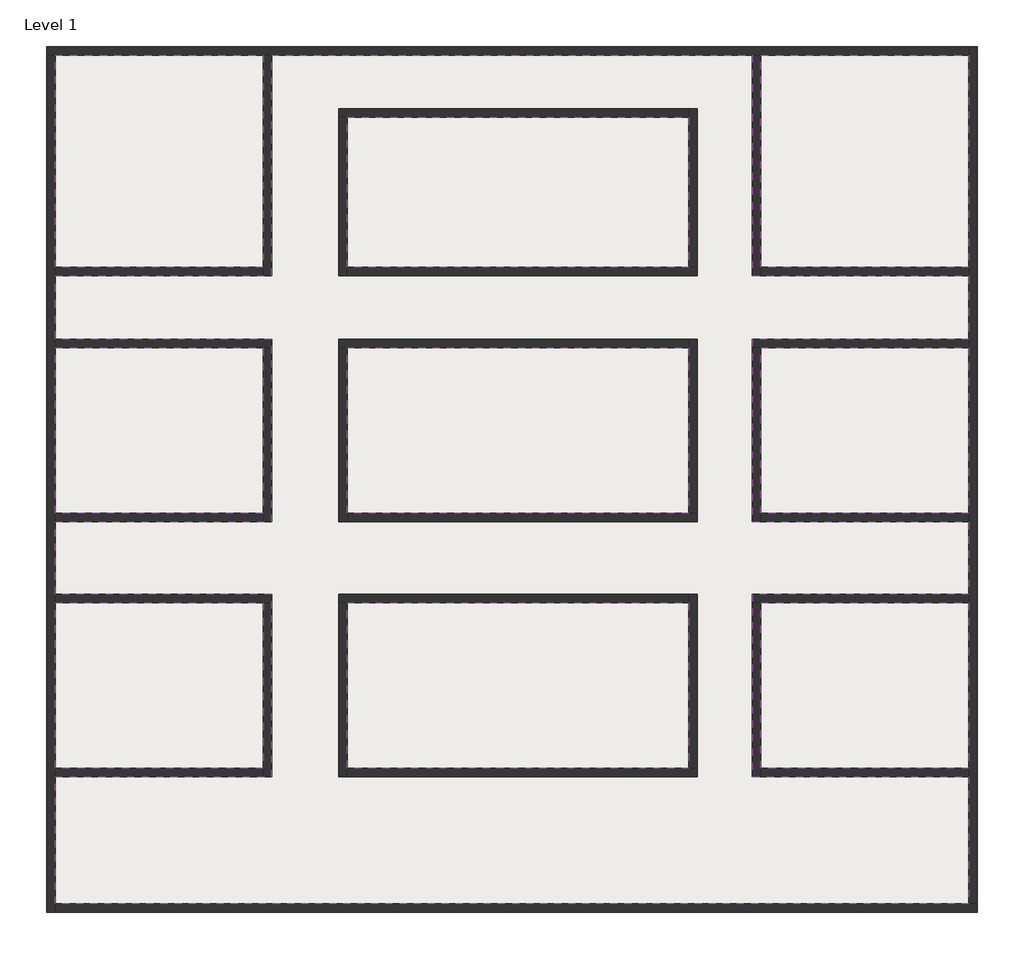
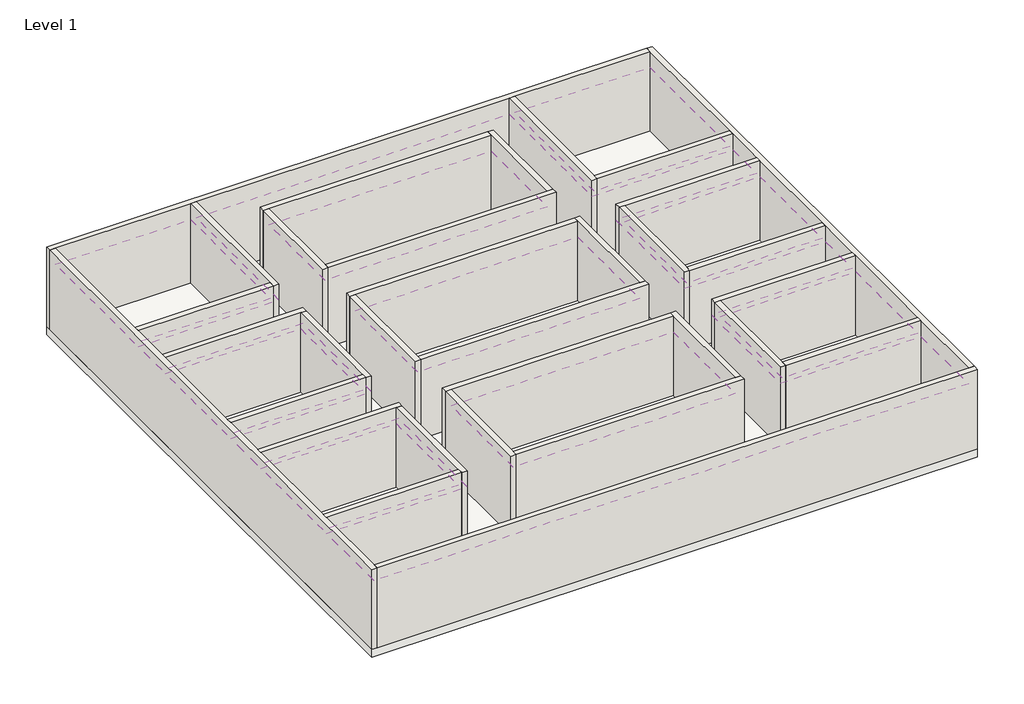
# One storey: 32 walls, 11 coverings, 1 slab.
"""IFC4 building model written with IfcOpenShell, lengths in millimetres."""

from ifc_helpers import new_model, si_unit, frame, origin, origin_with_axes, place, context, project, spatial, polyline, outline, extrude, faceted_brep, element, save

model = new_model("IFC4")

# Units and contexts
model_context = context("Model", 3, world=origin())
ifc_project = project(units=[si_unit("LENGTHUNIT", "METRE", prefix="MILLI")], contexts=[model_context])

# Site, building, storey
site = spatial("IfcSite", under=ifc_project)
building = spatial("IfcBuilding", under=site)
storey = spatial("IfcBuildingStorey", under=building, Name="Level 1", Elevation=0.0)

# Coverings
placement = place(None, origin())
element("IfcCovering", 1, ObjectType="2' x 4' ACT System", at=placement, inside=storey, context=model_context, shape_type="SweptSolid", body=[
    extrude(outline(polyline([(-11709.662063, 12460.3552234), (-6809.662063, 12460.3552234), (-6809.662063, 7460.3552234), (-11709.662063, 7460.3552234), (-11709.662063, 12460.3552234)])), frame((0.0, 0.0, 2438.4), z_axis=(0.0, 0.0, 1.0), x_axis=(1.0, 0.0, 0.0)), (0.0, 0.0, 1.0), 57.15),
])
element("IfcCovering", 2, ObjectType="2' x 4' ACT System", at=placement, inside=storey, context=model_context, shape_type="SweptSolid", body=[
    extrude(outline(polyline([(-6609.662063, 7260.3552234), (-6609.662063, 12460.3552234), (4722.664183, 12460.3552234), (4722.664183, 7260.3552234), (9822.664183, 7260.3552234), (9822.664183, 5760.3552234), (4722.664183, 5760.3552234), (4722.664183, 1460.3552234), (9822.664183, 1460.3552234), (9822.664183, -239.6447766), (4722.664183, -239.6447766), (4722.664183, -4539.6447766), (9822.664183, -4539.6447766), (9822.664183, -7539.6447766), (-11709.662063, -7539.6447766), (-11709.662063, -4539.6447766), (-6609.662063, -4539.6447766), (-6609.662063, -239.6447766), (-11709.662063, -239.6447766), (-11709.662063, 1460.3552234), (-6609.662063, 1460.3552234), (-6609.662063, 5760.3552234), (-11709.662063, 5760.3552234), (-11709.662063, 7260.3552234), (-6609.662063, 7260.3552234)]), holes=[polyline([(3422.664183, 7260.3552234), (3422.664183, 11191.3898121), (-5023.4293583, 11191.3898121), (-5023.4293583, 7260.3552234), (3422.664183, 7260.3552234)]), polyline([(3422.664183, 1460.3552234), (3422.664183, 5760.3552234), (-5023.4293583, 5760.3552234), (-5023.4293583, 1460.3552234), (3422.664183, 1460.3552234)]), polyline([(3422.664183, -4539.6447766), (3422.664183, -239.6447766), (-5023.4293583, -239.6447766), (-5023.4293583, -4539.6447766), (3422.664183, -4539.6447766)])]), frame((0.0, 0.0, 2438.4), z_axis=(0.0, 0.0, 1.0), x_axis=(1.0, 0.0, 0.0)), (0.0, 0.0, 1.0), 57.15),
])
element("IfcCovering", 3, ObjectType="2' x 4' ACT System", at=placement, inside=storey, context=model_context, shape_type="SweptSolid", body=[
    extrude(outline(polyline([(-4823.4293583, 10991.3898121), (3222.664183, 10991.3898121), (3222.664183, 7460.3552234), (-4823.4293583, 7460.3552234), (-4823.4293583, 10991.3898121)])), frame((0.0, 0.0, 2438.4), z_axis=(0.0, 0.0, 1.0), x_axis=(1.0, 0.0, 0.0)), (0.0, 0.0, 1.0), 57.15),
])
element("IfcCovering", 4, ObjectType="2' x 4' ACT System", at=placement, inside=storey, context=model_context, shape_type="SweptSolid", body=[
    extrude(outline(polyline([(4922.664183, 7460.3552234), (4922.664183, 12460.3552234), (9822.664183, 12460.3552234), (9822.664183, 7460.3552234), (4922.664183, 7460.3552234)])), frame((0.0, 0.0, 2438.4), z_axis=(0.0, 0.0, 1.0), x_axis=(1.0, 0.0, 0.0)), (0.0, 0.0, 1.0), 57.15),
])
element("IfcCovering", 5, ObjectType="2' x 4' ACT System", at=placement, inside=storey, context=model_context, shape_type="SweptSolid", body=[
    extrude(outline(polyline([(4922.664183, 5560.3552234), (9822.664183, 5560.3552234), (9822.664183, 1660.3552234), (4922.664183, 1660.3552234), (4922.664183, 5560.3552234)])), frame((0.0, 0.0, 2438.4), z_axis=(0.0, 0.0, 1.0), x_axis=(1.0, 0.0, 0.0)), (0.0, 0.0, 1.0), 57.15),
])
element("IfcCovering", 6, ObjectType="2' x 4' ACT System", at=placement, inside=storey, context=model_context, shape_type="SweptSolid", body=[
    extrude(outline(polyline([(4922.664183, -439.6447766), (9822.664183, -439.6447766), (9822.664183, -4339.6447766), (4922.664183, -4339.6447766), (4922.664183, -439.6447766)])), frame((0.0, 0.0, 2438.4), z_axis=(0.0, 0.0, 1.0), x_axis=(1.0, 0.0, 0.0)), (0.0, 0.0, 1.0), 57.15),
])
element("IfcCovering", 7, ObjectType="2' x 4' ACT System", at=placement, inside=storey, context=model_context, shape_type="SweptSolid", body=[
    extrude(outline(polyline([(-4823.4293583, -439.6447766), (3222.664183, -439.6447766), (3222.664183, -4339.6447766), (-4823.4293583, -4339.6447766), (-4823.4293583, -439.6447766)])), frame((0.0, 0.0, 2438.4), z_axis=(0.0, 0.0, 1.0), x_axis=(1.0, 0.0, 0.0)), (0.0, 0.0, 1.0), 57.15),
])
element("IfcCovering", 8, ObjectType="2' x 4' ACT System", at=placement, inside=storey, context=model_context, shape_type="SweptSolid", body=[
    extrude(outline(polyline([(-11709.662063, -4339.6447766), (-11709.662063, -439.6447766), (-6809.662063, -439.6447766), (-6809.662063, -4339.6447766), (-11709.662063, -4339.6447766)])), frame((0.0, 0.0, 2438.4), z_axis=(0.0, 0.0, 1.0), x_axis=(1.0, 0.0, 0.0)), (0.0, 0.0, 1.0), 57.15),
])
element("IfcCovering", 9, ObjectType="2' x 4' ACT System", at=placement, inside=storey, context=model_context, shape_type="SweptSolid", body=[
    extrude(outline(polyline([(-11709.662063, 1660.3552234), (-11709.662063, 5560.3552234), (-6809.662063, 5560.3552234), (-6809.662063, 1660.3552234), (-11709.662063, 1660.3552234)])), frame((0.0, 0.0, 2438.4), z_axis=(0.0, 0.0, 1.0), x_axis=(1.0, 0.0, 0.0)), (0.0, 0.0, 1.0), 57.15),
])
element("IfcCovering", 10, ObjectType="2' x 4' ACT System", at=placement, inside=storey, context=model_context, shape_type="SweptSolid", body=[
    extrude(outline(polyline([(-4823.4293583, 5560.3552234), (3222.664183, 5560.3552234), (3222.664183, 1660.3552234), (-4823.4293583, 1660.3552234), (-4823.4293583, 5560.3552234)])), frame((0.0, 0.0, 2438.4), z_axis=(0.0, 0.0, 1.0), x_axis=(1.0, 0.0, 0.0)), (0.0, 0.0, 1.0), 57.15),
])
element("IfcCovering", 11, ObjectType="2' x 4' ACT System", at=placement, inside=storey, context=model_context, shape_type="SweptSolid", body=[
    extrude(outline(polyline([(4922.664183, 5560.3552234), (9822.664183, 5560.3552234), (9822.664183, 1660.3552234), (4922.664183, 1660.3552234), (4922.664183, 5560.3552234)])), frame((0.0, 0.0, 2438.4), z_axis=(0.0, 0.0, 1.0), x_axis=(1.0, 0.0, 0.0)), (0.0, 0.0, 1.0), 57.15),
])

# Slab
element("IfcSlab", 12, ObjectType="Generic - 12\"", at=placement, inside=storey, context=model_context, shape_type="SweptSolid", body=[
    extrude(outline(polyline([(10022.664183, 12660.3552234), (10022.664183, -7739.6447766), (-11909.662063, -7739.6447766), (-11909.662063, 12660.3552234), (10022.664183, 12660.3552234)])), frame((0.0, 0.0, -304.8), z_axis=(0.0, 0.0, 1.0), x_axis=(1.0, 0.0, 0.0)), (0.0, 0.0, 1.0), 304.8),
])

# Walls
element("IfcWall", 13, ObjectType="Generic - 200mm", at=placement, inside=storey, context=model_context, shape_type="Brep", body=[
    faceted_brep([(-11909.662063, 12460.3552234, 0.0), (-11709.662063, 12460.3552234, 0.0), (-6809.662063, 12460.3552234, 0.0), (-6609.662063, 12460.3552234, 0.0), (4722.664183, 12460.3552234, 0.0), (4922.664183, 12460.3552234, 0.0), (9822.664183, 12460.3552234, 0.0), (9822.664183, 12460.3552234, 3048.0), (4922.664183, 12460.3552234, 3048.0), (4722.664183, 12460.3552234, 3048.0), (-6609.662063, 12460.3552234, 3048.0), (-6809.662063, 12460.3552234, 3048.0), (-11709.662063, 12460.3552234, 3048.0), (-11909.662063, 12460.3552234, 3048.0), (-11909.662063, 12660.3552234, 0.0), (-11909.662063, 12660.3552234, 3048.0), (9822.664183, 12660.3552234, 3048.0), (9822.664183, 12660.3552234, 0.0)], [[[0, 1, 2, 3, 4, 5, 6, 7, 8, 9, 10, 11, 12, 13]], [[14, 15, 16, 17]], [[6, 5, 4, 3, 2, 1, 0, 14, 17]], [[0, 13, 15, 14]], [[7, 6, 17, 16]], [[13, 12, 11, 10, 9, 8, 7, 16, 15]]]),
])
element("IfcWall", 14, ObjectType="Generic - 200mm", at=placement, inside=storey, context=model_context, shape_type="Brep", body=[
    faceted_brep([(-11709.662063, -7739.6447766, 0.0), (-11709.662063, -7539.6447766, 0.0), (-11709.662063, -4539.6447766, 0.0), (-11709.662063, -4339.6447766, 0.0), (-11709.662063, -439.6447766, 0.0), (-11709.662063, -239.6447766, 0.0), (-11709.662063, 1460.3552234, 0.0), (-11709.662063, 1660.3552234, 0.0), (-11709.662063, 5560.3552234, 0.0), (-11709.662063, 5760.3552234, 0.0), (-11709.662063, 7260.3552234, 0.0), (-11709.662063, 7460.3552234, 0.0), (-11709.662063, 12460.3552234, 0.0), (-11709.662063, 12460.3552234, 3048.0), (-11709.662063, 7460.3552234, 3048.0), (-11709.662063, 7260.3552234, 3048.0), (-11709.662063, 5760.3552234, 3048.0), (-11709.662063, 5560.3552234, 3048.0), (-11709.662063, 1660.3552234, 3048.0), (-11709.662063, 1460.3552234, 3048.0), (-11709.662063, -239.6447766, 3048.0), (-11709.662063, -439.6447766, 3048.0), (-11709.662063, -4339.6447766, 3048.0), (-11709.662063, -4539.6447766, 3048.0), (-11709.662063, -7539.6447766, 3048.0), (-11709.662063, -7739.6447766, 3048.0), (-11909.662063, -7739.6447766, 0.0), (-11909.662063, -7739.6447766, 3048.0), (-11909.662063, 12460.3552234, 3048.0), (-11909.662063, 12460.3552234, 0.0)], [[[0, 1, 2, 3, 4, 5, 6, 7, 8, 9, 10, 11, 12, 13, 14, 15, 16, 17, 18, 19, 20, 21, 22, 23, 24, 25]], [[26, 27, 28, 29]], [[12, 11, 10, 9, 8, 7, 6, 5, 4, 3, 2, 1, 0, 26, 29]], [[0, 25, 27, 26]], [[13, 12, 29, 28]], [[25, 24, 23, 22, 21, 20, 19, 18, 17, 16, 15, 14, 13, 28, 27]]]),
])
element("IfcWall", 15, ObjectType="Generic - 200mm", at=placement, inside=storey, context=model_context, shape_type="Brep", body=[
    faceted_brep([(10022.664183, -7539.6447766, 0.0), (9822.664183, -7539.6447766, 0.0), (-11709.662063, -7539.6447766, 0.0), (-11709.662063, -7539.6447766, 3048.0), (9822.664183, -7539.6447766, 3048.0), (10022.664183, -7539.6447766, 3048.0), (10022.664183, -7739.6447766, 0.0), (10022.664183, -7739.6447766, 3048.0), (-11709.662063, -7739.6447766, 3048.0), (-11709.662063, -7739.6447766, 0.0)], [[[0, 1, 2, 3, 4, 5]], [[6, 7, 8, 9]], [[2, 1, 0, 6, 9]], [[0, 5, 7, 6]], [[3, 2, 9, 8]], [[5, 4, 3, 8, 7]]]),
])
element("IfcWall", 16, ObjectType="Generic - 200mm", at=placement, inside=storey, context=model_context, shape_type="Brep", body=[
    faceted_brep([(9822.664183, 12660.3552234, 0.0), (9822.664183, 12460.3552234, 0.0), (9822.664183, 7460.3552234, 0.0), (9822.664183, 7260.3552234, 0.0), (9822.664183, 5760.3552234, 0.0), (9822.664183, 5560.3552234, 0.0), (9822.664183, 1660.3552234, 0.0), (9822.664183, 1460.3552234, 0.0), (9822.664183, -239.6447766, 0.0), (9822.664183, -439.6447766, 0.0), (9822.664183, -4339.6447766, 0.0), (9822.664183, -4539.6447766, 0.0), (9822.664183, -7539.6447766, 0.0), (9822.664183, -7539.6447766, 3048.0), (9822.664183, -4539.6447766, 3048.0), (9822.664183, -4339.6447766, 3048.0), (9822.664183, -439.6447766, 3048.0), (9822.664183, -239.6447766, 3048.0), (9822.664183, 1460.3552234, 3048.0), (9822.664183, 1660.3552234, 3048.0), (9822.664183, 5560.3552234, 3048.0), (9822.664183, 5760.3552234, 3048.0), (9822.664183, 7260.3552234, 3048.0), (9822.664183, 7460.3552234, 3048.0), (9822.664183, 12460.3552234, 3048.0), (9822.664183, 12660.3552234, 3048.0), (10022.664183, 12660.3552234, 0.0), (10022.664183, 12660.3552234, 3048.0), (10022.664183, -7539.6447766, 3048.0), (10022.664183, -7539.6447766, 0.0)], [[[0, 1, 2, 3, 4, 5, 6, 7, 8, 9, 10, 11, 12, 13, 14, 15, 16, 17, 18, 19, 20, 21, 22, 23, 24, 25]], [[26, 27, 28, 29]], [[12, 11, 10, 9, 8, 7, 6, 5, 4, 3, 2, 1, 0, 26, 29]], [[0, 25, 27, 26]], [[13, 12, 29, 28]], [[25, 24, 23, 22, 21, 20, 19, 18, 17, 16, 15, 14, 13, 28, 27]]]),
])
element("IfcWall", 17, ObjectType="Generic - 200mm", at=placement, inside=storey, context=model_context, shape_type="Brep", body=[
    faceted_brep([(-6809.662063, -439.6447766, 0.0), (-6809.662063, -4339.6447766, 0.0), (-6809.662063, -4539.6447766, 0.0), (-6809.662063, -4539.6447766, 3048.0), (-6809.662063, -4339.6447766, 3048.0), (-6809.662063, -439.6447766, 3048.0), (-6609.662063, -439.6447766, 0.0), (-6609.662063, -439.6447766, 3048.0), (-6609.662063, -4539.6447766, 3048.0), (-6609.662063, -4539.6447766, 0.0)], [[[0, 1, 2, 3, 4, 5]], [[6, 7, 8, 9]], [[2, 1, 0, 6, 9]], [[3, 2, 9, 8]], [[0, 5, 7, 6]], [[5, 4, 3, 8, 7]]]),
])
element("IfcWall", 18, ObjectType="Generic - 200mm", at=placement, inside=storey, context=model_context, shape_type="SweptSolid", body=[
    extrude(outline(polyline([(-11709.662063, -4339.6447766), (-6809.662063, -4339.6447766), (-6809.662063, -4539.6447766), (-11709.662063, -4539.6447766), (-11709.662063, -4339.6447766)])), origin_with_axes(), (0.0, 0.0, 1.0), 3048.0),
])
element("IfcWall", 19, ObjectType="Generic - 200mm", at=placement, inside=storey, context=model_context, shape_type="Brep", body=[
    faceted_brep([(-11709.662063, -439.6447766, 0.0), (-6809.662063, -439.6447766, 0.0), (-6609.662063, -439.6447766, 0.0), (-6609.662063, -439.6447766, 3048.0), (-6809.662063, -439.6447766, 3048.0), (-11709.662063, -439.6447766, 3048.0), (-11709.662063, -239.6447766, 0.0), (-11709.662063, -239.6447766, 3048.0), (-6609.662063, -239.6447766, 3048.0), (-6609.662063, -239.6447766, 0.0)], [[[0, 1, 2, 3, 4, 5]], [[6, 7, 8, 9]], [[2, 1, 0, 6, 9]], [[0, 5, 7, 6]], [[3, 2, 9, 8]], [[5, 4, 3, 8, 7]]]),
])
element("IfcWall", 20, ObjectType="Generic - 200mm", at=placement, inside=storey, context=model_context, shape_type="Brep", body=[
    faceted_brep([(-6809.662063, 5560.3552234, 0.0), (-6809.662063, 1660.3552234, 0.0), (-6809.662063, 1460.3552234, 0.0), (-6809.662063, 1460.3552234, 3048.0), (-6809.662063, 1660.3552234, 3048.0), (-6809.662063, 5560.3552234, 3048.0), (-6609.662063, 5560.3552234, 0.0), (-6609.662063, 5560.3552234, 3048.0), (-6609.662063, 1460.3552234, 3048.0), (-6609.662063, 1460.3552234, 0.0)], [[[0, 1, 2, 3, 4, 5]], [[6, 7, 8, 9]], [[2, 1, 0, 6, 9]], [[3, 2, 9, 8]], [[0, 5, 7, 6]], [[5, 4, 3, 8, 7]]]),
])
element("IfcWall", 21, ObjectType="Generic - 200mm", at=placement, inside=storey, context=model_context, shape_type="SweptSolid", body=[
    extrude(outline(polyline([(-11709.662063, 1660.3552234), (-6809.662063, 1660.3552234), (-6809.662063, 1460.3552234), (-11709.662063, 1460.3552234), (-11709.662063, 1660.3552234)])), origin_with_axes(), (0.0, 0.0, 1.0), 3048.0),
])
element("IfcWall", 22, ObjectType="Generic - 200mm", at=placement, inside=storey, context=model_context, shape_type="Brep", body=[
    faceted_brep([(-11709.662063, 5560.3552234, 0.0), (-6809.662063, 5560.3552234, 0.0), (-6609.662063, 5560.3552234, 0.0), (-6609.662063, 5560.3552234, 3048.0), (-6809.662063, 5560.3552234, 3048.0), (-11709.662063, 5560.3552234, 3048.0), (-11709.662063, 5760.3552234, 0.0), (-11709.662063, 5760.3552234, 3048.0), (-6609.662063, 5760.3552234, 3048.0), (-6609.662063, 5760.3552234, 0.0)], [[[0, 1, 2, 3, 4, 5]], [[6, 7, 8, 9]], [[2, 1, 0, 6, 9]], [[3, 2, 9, 8]], [[0, 5, 7, 6]], [[5, 4, 3, 8, 7]]]),
])
element("IfcWall", 23, ObjectType="Generic - 200mm", at=placement, inside=storey, context=model_context, shape_type="Brep", body=[
    faceted_brep([(-6809.662063, 12460.3552234, 0.0), (-6809.662063, 7460.3552234, 0.0), (-6809.662063, 7260.3552234, 0.0), (-6809.662063, 7260.3552234, 3048.0), (-6809.662063, 7460.3552234, 3048.0), (-6809.662063, 12460.3552234, 3048.0), (-6609.662063, 12460.3552234, 0.0), (-6609.662063, 12460.3552234, 3048.0), (-6609.662063, 7260.3552234, 3048.0), (-6609.662063, 7260.3552234, 0.0)], [[[0, 1, 2, 3, 4, 5]], [[6, 7, 8, 9]], [[2, 1, 0, 6, 9]], [[3, 2, 9, 8]], [[0, 5, 7, 6]], [[5, 4, 3, 8, 7]]]),
])
element("IfcWall", 24, ObjectType="Generic - 200mm", at=placement, inside=storey, context=model_context, shape_type="SweptSolid", body=[
    extrude(outline(polyline([(-11709.662063, 7460.3552234), (-6809.662063, 7460.3552234), (-6809.662063, 7260.3552234), (-11709.662063, 7260.3552234), (-11709.662063, 7460.3552234)])), origin_with_axes(), (0.0, 0.0, 1.0), 3048.0),
])
element("IfcWall", 25, ObjectType="Generic - 200mm", at=placement, inside=storey, context=model_context, shape_type="Brep", body=[
    faceted_brep([(-5023.4293583, 10991.3898121, 0.0), (-4823.4293583, 10991.3898121, 0.0), (3222.664183, 10991.3898121, 0.0), (3222.664183, 10991.3898121, 3048.0), (-4823.4293583, 10991.3898121, 3048.0), (-5023.4293583, 10991.3898121, 3048.0), (-5023.4293583, 11191.3898121, 0.0), (-5023.4293583, 11191.3898121, 3048.0), (3222.664183, 11191.3898121, 3048.0), (3222.664183, 11191.3898121, 0.0)], [[[0, 1, 2, 3, 4, 5]], [[6, 7, 8, 9]], [[2, 1, 0, 6, 9]], [[0, 5, 7, 6]], [[3, 2, 9, 8]], [[5, 4, 3, 8, 7]]]),
])
element("IfcWall", 26, ObjectType="Generic - 200mm", at=placement, inside=storey, context=model_context, shape_type="Brep", body=[
    faceted_brep([(-4823.4293583, 7260.3552234, 0.0), (-4823.4293583, 7460.3552234, 0.0), (-4823.4293583, 10991.3898121, 0.0), (-4823.4293583, 10991.3898121, 3048.0), (-4823.4293583, 7460.3552234, 3048.0), (-4823.4293583, 7260.3552234, 3048.0), (-5023.4293583, 7260.3552234, 0.0), (-5023.4293583, 7260.3552234, 3048.0), (-5023.4293583, 10991.3898121, 3048.0), (-5023.4293583, 10991.3898121, 0.0)], [[[0, 1, 2, 3, 4, 5]], [[6, 7, 8, 9]], [[2, 1, 0, 6, 9]], [[0, 5, 7, 6]], [[3, 2, 9, 8]], [[5, 4, 3, 8, 7]]]),
])
element("IfcWall", 27, ObjectType="Generic - 200mm", at=placement, inside=storey, context=model_context, shape_type="Brep", body=[
    faceted_brep([(3422.664183, 7460.3552234, 0.0), (3222.664183, 7460.3552234, 0.0), (-4823.4293583, 7460.3552234, 0.0), (-4823.4293583, 7460.3552234, 3048.0), (3222.664183, 7460.3552234, 3048.0), (3422.664183, 7460.3552234, 3048.0), (3422.664183, 7260.3552234, 0.0), (3422.664183, 7260.3552234, 3048.0), (-4823.4293583, 7260.3552234, 3048.0), (-4823.4293583, 7260.3552234, 0.0)], [[[0, 1, 2, 3, 4, 5]], [[6, 7, 8, 9]], [[2, 1, 0, 6, 9]], [[0, 5, 7, 6]], [[3, 2, 9, 8]], [[5, 4, 3, 8, 7]]]),
])
element("IfcWall", 28, ObjectType="Generic - 200mm", at=placement, inside=storey, context=model_context, shape_type="Brep", body=[
    faceted_brep([(3222.664183, 11191.3898121, 0.0), (3222.664183, 10991.3898121, 0.0), (3222.664183, 7460.3552234, 0.0), (3222.664183, 7460.3552234, 3048.0), (3222.664183, 10991.3898121, 3048.0), (3222.664183, 11191.3898121, 3048.0), (3422.664183, 11191.3898121, 0.0), (3422.664183, 11191.3898121, 3048.0), (3422.664183, 7460.3552234, 3048.0), (3422.664183, 7460.3552234, 0.0)], [[[0, 1, 2, 3, 4, 5]], [[6, 7, 8, 9]], [[2, 1, 0, 6, 9]], [[0, 5, 7, 6]], [[3, 2, 9, 8]], [[5, 4, 3, 8, 7]]]),
])
element("IfcWall", 29, ObjectType="Generic - 200mm", at=placement, inside=storey, context=model_context, shape_type="Brep", body=[
    faceted_brep([(-5023.4293583, 5560.3552234, 0.0), (-4823.4293583, 5560.3552234, 0.0), (3222.664183, 5560.3552234, 0.0), (3222.664183, 5560.3552234, 3048.0), (-4823.4293583, 5560.3552234, 3048.0), (-5023.4293583, 5560.3552234, 3048.0), (-5023.4293583, 5760.3552234, 0.0), (-5023.4293583, 5760.3552234, 3048.0), (3222.664183, 5760.3552234, 3048.0), (3222.664183, 5760.3552234, 0.0)], [[[0, 1, 2, 3, 4, 5]], [[6, 7, 8, 9]], [[2, 1, 0, 6, 9]], [[0, 5, 7, 6]], [[3, 2, 9, 8]], [[5, 4, 3, 8, 7]]]),
])
element("IfcWall", 30, ObjectType="Generic - 200mm", at=placement, inside=storey, context=model_context, shape_type="Brep", body=[
    faceted_brep([(-4823.4293583, 1460.3552234, 0.0), (-4823.4293583, 1660.3552234, 0.0), (-4823.4293583, 5560.3552234, 0.0), (-4823.4293583, 5560.3552234, 3048.0), (-4823.4293583, 1660.3552234, 3048.0), (-4823.4293583, 1460.3552234, 3048.0), (-5023.4293583, 1460.3552234, 0.0), (-5023.4293583, 1460.3552234, 3048.0), (-5023.4293583, 5560.3552234, 3048.0), (-5023.4293583, 5560.3552234, 0.0)], [[[0, 1, 2, 3, 4, 5]], [[6, 7, 8, 9]], [[2, 1, 0, 6, 9]], [[0, 5, 7, 6]], [[3, 2, 9, 8]], [[5, 4, 3, 8, 7]]]),
])
element("IfcWall", 31, ObjectType="Generic - 200mm", at=placement, inside=storey, context=model_context, shape_type="Brep", body=[
    faceted_brep([(3422.664183, 1660.3552234, 0.0), (3222.664183, 1660.3552234, 0.0), (-4823.4293583, 1660.3552234, 0.0), (-4823.4293583, 1660.3552234, 3048.0), (3222.664183, 1660.3552234, 3048.0), (3422.664183, 1660.3552234, 3048.0), (3422.664183, 1460.3552234, 0.0), (3422.664183, 1460.3552234, 3048.0), (-4823.4293583, 1460.3552234, 3048.0), (-4823.4293583, 1460.3552234, 0.0)], [[[0, 1, 2, 3, 4, 5]], [[6, 7, 8, 9]], [[2, 1, 0, 6, 9]], [[0, 5, 7, 6]], [[3, 2, 9, 8]], [[5, 4, 3, 8, 7]]]),
])
element("IfcWall", 32, ObjectType="Generic - 200mm", at=placement, inside=storey, context=model_context, shape_type="Brep", body=[
    faceted_brep([(3222.664183, 5760.3552234, 0.0), (3222.664183, 5560.3552234, 0.0), (3222.664183, 1660.3552234, 0.0), (3222.664183, 1660.3552234, 3048.0), (3222.664183, 5560.3552234, 3048.0), (3222.664183, 5760.3552234, 3048.0), (3422.664183, 5760.3552234, 0.0), (3422.664183, 5760.3552234, 3048.0), (3422.664183, 1660.3552234, 3048.0), (3422.664183, 1660.3552234, 0.0)], [[[0, 1, 2, 3, 4, 5]], [[6, 7, 8, 9]], [[2, 1, 0, 6, 9]], [[0, 5, 7, 6]], [[3, 2, 9, 8]], [[5, 4, 3, 8, 7]]]),
])
element("IfcWall", 33, ObjectType="Generic - 200mm", at=placement, inside=storey, context=model_context, shape_type="Brep", body=[
    faceted_brep([(-5023.4293583, -439.6447766, 0.0), (-4823.4293583, -439.6447766, 0.0), (3222.664183, -439.6447766, 0.0), (3222.664183, -439.6447766, 3048.0), (-4823.4293583, -439.6447766, 3048.0), (-5023.4293583, -439.6447766, 3048.0), (-5023.4293583, -239.6447766, 0.0), (-5023.4293583, -239.6447766, 3048.0), (3222.664183, -239.6447766, 3048.0), (3222.664183, -239.6447766, 0.0)], [[[0, 1, 2, 3, 4, 5]], [[6, 7, 8, 9]], [[2, 1, 0, 6, 9]], [[0, 5, 7, 6]], [[3, 2, 9, 8]], [[5, 4, 3, 8, 7]]]),
])
element("IfcWall", 34, ObjectType="Generic - 200mm", at=placement, inside=storey, context=model_context, shape_type="Brep", body=[
    faceted_brep([(-4823.4293583, -4539.6447766, 0.0), (-4823.4293583, -4339.6447766, 0.0), (-4823.4293583, -439.6447766, 0.0), (-4823.4293583, -439.6447766, 3048.0), (-4823.4293583, -4339.6447766, 3048.0), (-4823.4293583, -4539.6447766, 3048.0), (-5023.4293583, -4539.6447766, 0.0), (-5023.4293583, -4539.6447766, 3048.0), (-5023.4293583, -439.6447766, 3048.0), (-5023.4293583, -439.6447766, 0.0)], [[[0, 1, 2, 3, 4, 5]], [[6, 7, 8, 9]], [[2, 1, 0, 6, 9]], [[0, 5, 7, 6]], [[3, 2, 9, 8]], [[5, 4, 3, 8, 7]]]),
])
element("IfcWall", 35, ObjectType="Generic - 200mm", at=placement, inside=storey, context=model_context, shape_type="Brep", body=[
    faceted_brep([(3422.664183, -4339.6447766, 0.0), (3222.664183, -4339.6447766, 0.0), (-4823.4293583, -4339.6447766, 0.0), (-4823.4293583, -4339.6447766, 3048.0), (3222.664183, -4339.6447766, 3048.0), (3422.664183, -4339.6447766, 3048.0), (3422.664183, -4539.6447766, 0.0), (3422.664183, -4539.6447766, 3048.0), (-4823.4293583, -4539.6447766, 3048.0), (-4823.4293583, -4539.6447766, 0.0)], [[[0, 1, 2, 3, 4, 5]], [[6, 7, 8, 9]], [[2, 1, 0, 6, 9]], [[0, 5, 7, 6]], [[3, 2, 9, 8]], [[5, 4, 3, 8, 7]]]),
])
element("IfcWall", 36, ObjectType="Generic - 200mm", at=placement, inside=storey, context=model_context, shape_type="Brep", body=[
    faceted_brep([(3222.664183, -239.6447766, 0.0), (3222.664183, -439.6447766, 0.0), (3222.664183, -4339.6447766, 0.0), (3222.664183, -4339.6447766, 3048.0), (3222.664183, -439.6447766, 3048.0), (3222.664183, -239.6447766, 3048.0), (3422.664183, -239.6447766, 0.0), (3422.664183, -239.6447766, 3048.0), (3422.664183, -4339.6447766, 3048.0), (3422.664183, -4339.6447766, 0.0)], [[[0, 1, 2, 3, 4, 5]], [[6, 7, 8, 9]], [[2, 1, 0, 6, 9]], [[0, 5, 7, 6]], [[3, 2, 9, 8]], [[5, 4, 3, 8, 7]]]),
])
element("IfcWall", 37, ObjectType="Generic - 200mm", at=placement, inside=storey, context=model_context, shape_type="Brep", body=[
    faceted_brep([(4722.664183, -439.6447766, 0.0), (4722.664183, -4539.6447766, 0.0), (4722.664183, -4539.6447766, 3048.0), (4722.664183, -439.6447766, 3048.0), (4922.664183, -439.6447766, 0.0), (4922.664183, -439.6447766, 3048.0), (4922.664183, -4339.6447766, 3048.0), (4922.664183, -4539.6447766, 3048.0), (4922.664183, -4539.6447766, 0.0), (4922.664183, -4339.6447766, 0.0)], [[[0, 1, 2, 3]], [[4, 5, 6, 7, 8, 9]], [[1, 0, 4, 9, 8]], [[2, 1, 8, 7]], [[0, 3, 5, 4]], [[3, 2, 7, 6, 5]]]),
])
element("IfcWall", 38, ObjectType="Generic - 200mm", at=placement, inside=storey, context=model_context, shape_type="SweptSolid", body=[
    extrude(outline(polyline([(9822.664183, -4539.6447766), (4922.664183, -4539.6447766), (4922.664183, -4339.6447766), (9822.664183, -4339.6447766), (9822.664183, -4539.6447766)])), origin_with_axes(), (0.0, 0.0, 1.0), 3048.0),
])
element("IfcWall", 39, ObjectType="Generic - 200mm", at=placement, inside=storey, context=model_context, shape_type="Brep", body=[
    faceted_brep([(9822.664183, -239.6447766, 0.0), (4722.664183, -239.6447766, 0.0), (4722.664183, -239.6447766, 3048.0), (9822.664183, -239.6447766, 3048.0), (9822.664183, -439.6447766, 0.0), (9822.664183, -439.6447766, 3048.0), (4922.664183, -439.6447766, 3048.0), (4722.664183, -439.6447766, 3048.0), (4722.664183, -439.6447766, 0.0), (4922.664183, -439.6447766, 0.0)], [[[0, 1, 2, 3]], [[4, 5, 6, 7, 8, 9]], [[1, 0, 4, 9, 8]], [[2, 1, 8, 7]], [[0, 3, 5, 4]], [[3, 2, 7, 6, 5]]]),
])
element("IfcWall", 40, ObjectType="Generic - 200mm", at=placement, inside=storey, context=model_context, shape_type="Brep", body=[
    faceted_brep([(4722.664183, 5560.3552234, 0.0), (4722.664183, 1460.3552234, 0.0), (4722.664183, 1460.3552234, 3048.0), (4722.664183, 5560.3552234, 3048.0), (4922.664183, 5560.3552234, 0.0), (4922.664183, 5560.3552234, 3048.0), (4922.664183, 1660.3552234, 3048.0), (4922.664183, 1460.3552234, 3048.0), (4922.664183, 1460.3552234, 0.0), (4922.664183, 1660.3552234, 0.0)], [[[0, 1, 2, 3]], [[4, 5, 6, 7, 8, 9]], [[1, 0, 4, 9, 8]], [[2, 1, 8, 7]], [[0, 3, 5, 4]], [[3, 2, 7, 6, 5]]]),
])
element("IfcWall", 41, ObjectType="Generic - 200mm", at=placement, inside=storey, context=model_context, shape_type="SweptSolid", body=[
    extrude(outline(polyline([(9822.664183, 1460.3552234), (4922.664183, 1460.3552234), (4922.664183, 1660.3552234), (9822.664183, 1660.3552234), (9822.664183, 1460.3552234)])), origin_with_axes(), (0.0, 0.0, 1.0), 3048.0),
])
element("IfcWall", 42, ObjectType="Generic - 200mm", at=placement, inside=storey, context=model_context, shape_type="Brep", body=[
    faceted_brep([(9822.664183, 5760.3552234, 0.0), (4722.664183, 5760.3552234, 0.0), (4722.664183, 5760.3552234, 3048.0), (9822.664183, 5760.3552234, 3048.0), (9822.664183, 5560.3552234, 0.0), (9822.664183, 5560.3552234, 3048.0), (4922.664183, 5560.3552234, 3048.0), (4722.664183, 5560.3552234, 3048.0), (4722.664183, 5560.3552234, 0.0), (4922.664183, 5560.3552234, 0.0)], [[[0, 1, 2, 3]], [[4, 5, 6, 7, 8, 9]], [[1, 0, 4, 9, 8]], [[2, 1, 8, 7]], [[0, 3, 5, 4]], [[3, 2, 7, 6, 5]]]),
])
element("IfcWall", 43, ObjectType="Generic - 200mm", at=placement, inside=storey, context=model_context, shape_type="Brep", body=[
    faceted_brep([(4722.664183, 12460.3552234, 0.0), (4722.664183, 7260.3552234, 0.0), (4722.664183, 7260.3552234, 3048.0), (4722.664183, 12460.3552234, 3048.0), (4922.664183, 12460.3552234, 0.0), (4922.664183, 12460.3552234, 3048.0), (4922.664183, 7460.3552234, 3048.0), (4922.664183, 7260.3552234, 3048.0), (4922.664183, 7260.3552234, 0.0), (4922.664183, 7460.3552234, 0.0)], [[[0, 1, 2, 3]], [[4, 5, 6, 7, 8, 9]], [[1, 0, 4, 9, 8]], [[2, 1, 8, 7]], [[0, 3, 5, 4]], [[3, 2, 7, 6, 5]]]),
])
element("IfcWall", 44, ObjectType="Generic - 200mm", at=placement, inside=storey, context=model_context, shape_type="SweptSolid", body=[
    extrude(outline(polyline([(9822.664183, 7260.3552234), (4922.664183, 7260.3552234), (4922.664183, 7460.3552234), (9822.664183, 7460.3552234), (9822.664183, 7260.3552234)])), origin_with_axes(), (0.0, 0.0, 1.0), 3048.0),
])

save(model, "model.ifc")

# Revit data of these elements
# Project information
#   Project Issue Date = "Issue Date"
#   Project Status = "Project Status"
#   Client Name = "Owner"
#   Project Address = "Enter address here"
#   Project Name = "Project Name"
#   Project Number = "Project Number"
# Type "2' x 4' ACT System"
#   Assembly Code = "C3030210"
#   built-in parameter 1002203 = 1 (stored number, unit not read)
#   built-in parameter 1002202 = 1 (stored number, unit not read)
#   Layers, outside or top first: 0.041275 m "Default" (function 1); 0.015875 m "Acoustic Ceiling Tile 24 x 48" (function 5)
# Type "Generic - 12\""
#   Assembly Code = "B1010"
#   Function = 0
#   Layers, outside or top first: 0.3048 m no material (function 1)
# Type "Generic - 200mm"
#   Layers, outside or top first: 0.2 m no material (function 1)
# Elements 1, 2, 3, 4, 5, 6, 7, 8, 9, 10, 11 (IfcCovering, "2' x 4' ACT System")
#   Height Offset From Level = 2.4384 m
#   Phase Created = New Construction
#   Materials on its faces: "Acoustic Ceiling Tile 24 x 48", "Default"
# Element 12 (IfcSlab, "Generic - 12\"")
#   Height Offset From Level = 0 m
#   Phase Created = New Construction
#   Materials on its faces: "Default Floor"
# Elements 13, 14, 15, 16, 17, 18, 19, 20, 21, 22, 23, 24, 25, 26, 27, 28, 29, 30, 31, 32, 33, 34, 35, 36, 37, 38, 39, 40, 41, 42, 43, 44 (IfcWall, "Generic - 200mm")
#   Top Offset = 0 m
#   Base Offset = 0 m
#   Unconnected Height = 3 m
#   wall height = 3 m
#   Phase Created = New Construction
#   Base Constraint = Level 1
#   Materials on its faces: "Default Wall"
# Materials
#   "Default": class "Miscellaneous", colour RGB 127 127 127, transparency 0, Cost = 0
#   "Acoustic Ceiling Tile 24 x 48": class "Generic", colour RGB 229 229 229, transparency 0, Description = "Acoustic Ceiling Tile 24 x 48", Cost = 0
#   "Default Floor": class "Miscellaneous", colour RGB 128 128 128, transparency 0, Cost = 0
#   "Default Wall": class "Miscellaneous", colour RGB 128 128 128, transparency 0, Cost = 0
